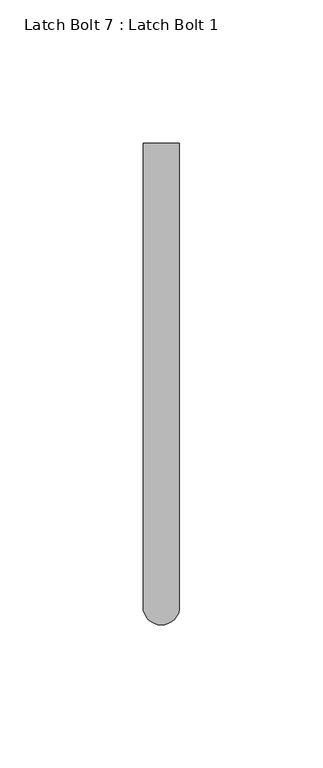
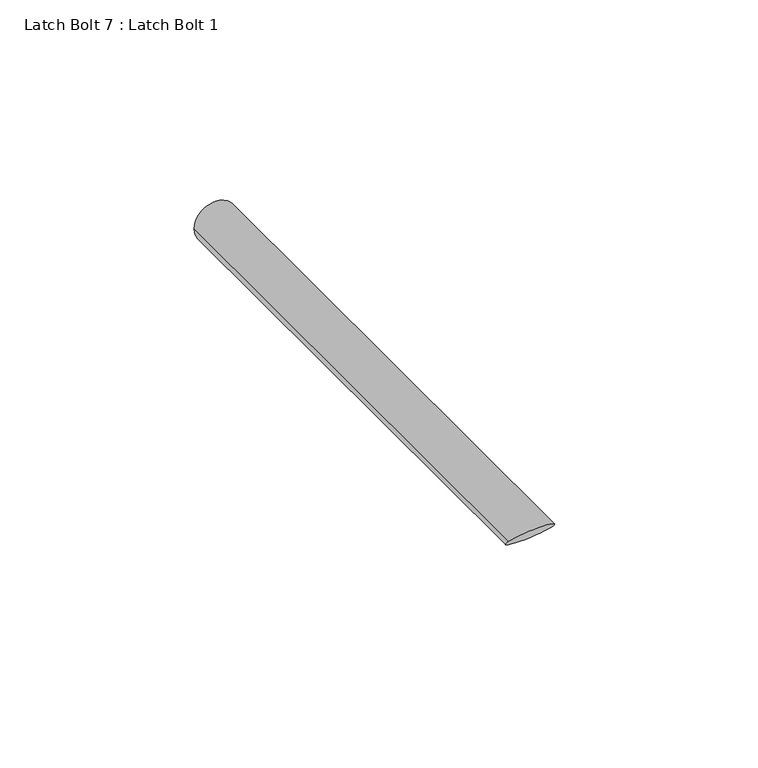
"""IFC4 building model written with IfcOpenShell, lengths in millimetres: proxy geometry, Latch Bolt 7 : Latch Bolt 1."""

from ifc_helpers import new_model, si_unit, frame, origin, place, context, project, spatial, circle_curve, ellipse_curve, source, transform, mapped, element, save
from ifc_brep_helpers import plane_surface, cylinder_surface, advanced_brep


def latch_bolt_7_latch_bolt_1_d9de4a67(model_context):
    return source(origin(), model_context, "Body", "AdvancedBrep", [
        advanced_brep(
        [(587306.3685739, -532807.6163841, 1066.8), (587319.0685739, -532807.6163841, 1066.8), (587306.3685739, -532969.5413841, 1066.8), (587312.7185739, -532975.8913841, 1073.15), (587319.0685739, -532969.5413841, 1066.8)],
        [
            (0, 1, circle_curve(frame((587312.7185739, -532807.6163841, 1066.8), z_axis=(0.0, 1.0, 0.0), x_axis=(1.0, 0.0, 0.0)), 6.35)),
            (1, 0, circle_curve(frame((587312.7185739, -532807.6163841, 1066.8), z_axis=(0.0, 1.0, 0.0), x_axis=(1.0, 0.0, 0.0)), 6.35)),
            (0, 2),
            (2, 3, ellipse_curve(frame((587312.7185739, -532969.5413841, 1066.8), z_axis=(0.0, 0.7071067811870104, 0.7071067811860847), x_axis=(0.0, 0.7071067811860846, -0.7071067811870104)), 8.9802561, 6.35)),
            (3, 4, ellipse_curve(frame((587312.7185739, -532969.5413841, 1066.8), z_axis=(0.0, 0.7071067811870104, 0.7071067811860847), x_axis=(0.0, 0.7071067811860846, -0.7071067811870104)), 8.9802561, 6.35)),
            (4, 1),
            (4, 2, ellipse_curve(frame((587312.7185739, -532969.5413841, 1066.8), z_axis=(0.0, 0.7071067811870104, 0.7071067811860847), x_axis=(0.0, 0.7071067811860846, -0.7071067811870104)), 8.9802561, 6.35)),
        ],
        [
            plane_surface(frame((587319.0685739, -532807.6163841, 1066.8), z_axis=(0.0, 1.0, 0.0), x_axis=(0.0, 0.0, -1.0))),
            cylinder_surface(frame((587312.7185739, -532975.8913841, 1066.8), z_axis=(0.0, 1.0, 0.0), x_axis=(1.0, 0.0, 0.0)), 6.35),
            plane_surface(frame((587338.1185739, -532960.0163841, 1057.275), z_axis=(0.0, -0.7071067811870104, -0.7071067811860847), x_axis=(-1.0, 0.0, 0.0))),
        ],
        [
            (0, [[1, 2]]),
            (1, [[-1, 3, 4, 5, 6]]),
            (1, [[-2, -6, 7, -3]]),
            (2, [[-4, -7, -5]]),
        ],
    ),
    ])


if __name__ == "__main__":
    model = new_model("IFC4")
    model_context = context("Model", 3, world=origin())
    ifc_project = project(units=[si_unit("LENGTHUNIT", "METRE", prefix="MILLI")], contexts=[model_context])
    site = spatial("IfcSite", under=ifc_project)
    building = spatial("IfcBuilding", under=site)
    placement = place(None, origin())
    latch_bolt_7_latch_bolt_1_shape = latch_bolt_7_latch_bolt_1_d9de4a67(model_context)
    element("IfcBuildingElementProxy", 1, Name="Latch Bolt 7 : Latch Bolt 1", ObjectType="Latch Bolt 7 : Latch Bolt 1", at=placement, inside=building, context=model_context, shape_type="MappedRepresentation", body=[
        mapped(latch_bolt_7_latch_bolt_1_shape, transform((0.0, 0.0, 0.0), x_axis=(1.0, 0.0, 0.0), y_axis=(0.0, 1.0, 0.0), z_axis=(0.0, 0.0, 1.0))),
    ])
    save(model, "model.ifc")

# Revit data of these elements
# Element 1 (IfcBuildingElementProxy, "Latch Bolt 7 : Latch Bolt 1")
#   Materials on its faces: "GALV. GATE LATCH"
# Materials
#   "GALV. GATE LATCH": class "Metal", colour RGB 189 187 185, transparency 0, Description = "Carbon steel", Cost = 0
